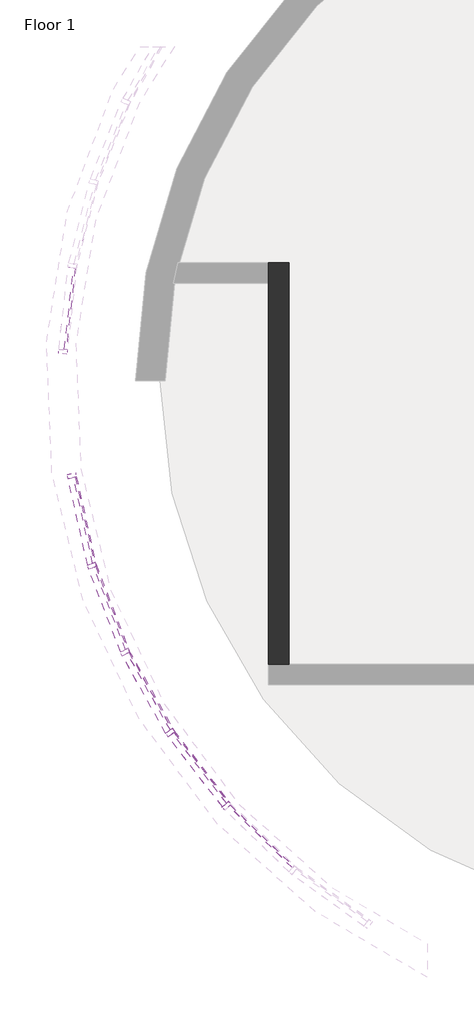
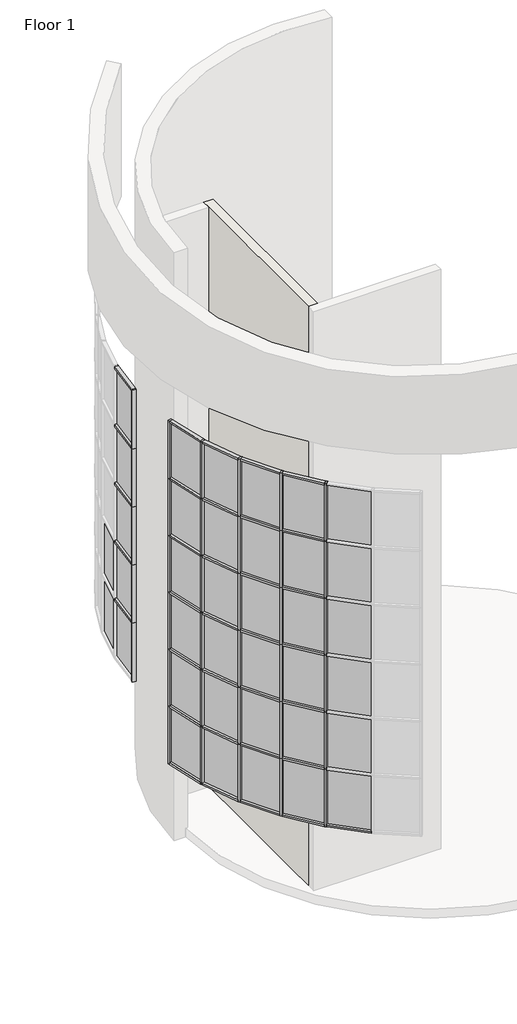
# One storey, part 1 of 11: 69 members, 37 plates, 1 wall.
# Revit data of these elements (continued)
# Type "Rectangular Mullion1 : 2.5\" x 5\" rectangular"
#   built-in parameter 1007304 = 0.416667 (stored number, unit not read)
#   built-in parameter 1007301 = 0.104167 (stored number, unit not read)
#   built-in parameter 1007300 = 0.104167 (stored number, unit not read)
# Type "System Panel : Glazed"
#   Construction Type Id = "GSP4R"
#   Analytic Construction = "1/8 in Pilkington single glazing"
#   Visual Light Transmittance = 0.9
#   Solar Heat Gain Coefficient = 0.86
#   Heat Transfer Coefficient (U) = 1.18115 BTU/(h·ft²·°F)
#   Define Thermal Properties by = 1
# Type "a_Mtl panel on Mtl stud"
#   Layers, outside or top first: 0' - 2" "Metal - Panel" (function 0); 0' - 3" "Misc. Air Layers - Air Space" (function 0); 0' - 0" "Air Barrier - Air Infiltration Barrier" (function 0); 0' - 0 3/4" "Wood - Sheathing - plywood" (function 0); 0' - 6" "Metal - Stud Layer" (function 0); 0' - 0" "Vapor / Moisture Barriers - Vapor Retarder" (function 0); 0' - 0 1/2" no material (function 0)
# Elements 1, 2, 3, 4, 5, 6, 7, 8, 9, 10, 11, 12, 13, 14, 15, 16, 17, 18, 19, 20, 21, 22, 23, 24, 25, 26, 27, 28, 29, 30, 31, 32, 33, 34, 35, 36, 37, 38, 39, 40, 41, 42, 43, 44, 45, 46, 47, 48, 49, 50, 51, 52, 53, 54, 55, 56, 57, 58, 59, 60, 61, 62, 63, 64, 65, 66, 67, 68, 69 (IfcMember, "Rectangular Mullion1 : 2.5\" x 5\" rectangular")
#   Phase Created = New Construction
#   Materials on its faces: "support-frame"
# Elements 70, 71, 72, 73, 74, 75, 76, 77, 78, 79, 80, 81, 82, 83, 84, 85, 86, 87, 88, 89, 90, 91, 92, 93, 94, 95, 96, 97, 98, 99, 100, 101, 102, 103, 104, 105, 106 (IfcPlate, "System Panel : Glazed")
#   Phase Created = New Construction
#   Materials on its faces: "Glass"
# Element 107 (IfcWall, "a_Mtl panel on Mtl stud")
#   Top Offset = 0' - 0"
#   Base Offset = 0' - 0"
#   wall height = 67' - 6"
#   Phase Created = New Construction
#   Base Constraint = Floor 1
#   Top Constraint = Parapet
#   Materials on its faces: "Default Wall", "Metal - Panel"
# Materials
#   "Metal - Panel": class "Unassigned", colour RGB 127 127 127, transparency 0
#   "Misc. Air Layers - Air Space": class "Miscellaneous", colour RGB 255 255 255, transparency 0
#   "Air Barrier - Air Infiltration Barrier": class "Miscellaneous", colour RGB 127 127 127, transparency 0
#   "Wood - Sheathing - plywood": class "Wood", colour RGB 212 179 113, transparency 0
#   "Metal - Stud Layer": class "Metal", colour RGB 199 199 199, transparency 0
#   "Vapor / Moisture Barriers - Vapor Retarder": class "Miscellaneous", colour RGB 127 127 127, transparency 0
#   "support-frame": class "Unassigned", colour RGB 233 233 233, transparency 0, Cost = 0
#   "Glass": class "Glass", colour RGB 0 128 192, transparency 0.75, Description = "Soda Lime Glass", Cost = 0
#   "Default Wall": class "Miscellaneous", colour RGB 128 128 128, transparency 0, Cost = 0
# Area at (34700.857, 51318.187) mm, upper offset 8' - 0", lower offset 0' - 0"
#   Number = "18"
#   Name = "Office Space"
# Area at (49006.684, 46244.199) mm, upper offset 8' - 0", lower offset 0' - 0"
#   Number = "19"
#   Name = "Core"
# Area at (1629.398, 48902.392) mm, upper offset 8' - 0", lower offset 0' - 0"
#   Number = "20"
#   Name = "Core"
# Area at (-5186.325, 48217.417) mm, upper offset 8' - 0", lower offset 0' - 0"
#   Number = "21"
#   Name = "Circulation"
# Area at (-13783.915, 48217.417) mm, upper offset 8' - 0", lower offset 0' - 0"
#   Number = "22"
#   Name = "Atrium"
# Area at (6186.704, 21308.019) mm, upper offset 8' - 0", lower offset 0' - 0"
#   Number = "23"
#   Name = "Office Space"
